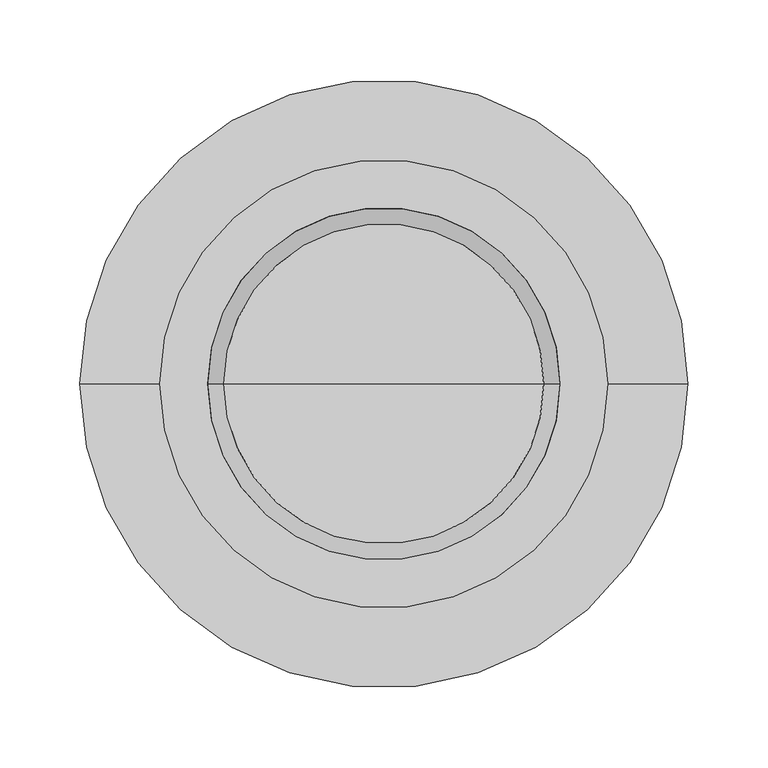
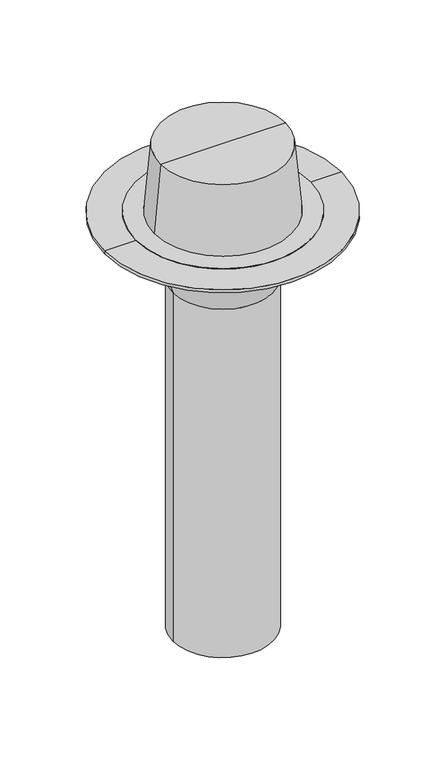
"""IFC4 building model written with IfcOpenShell, lengths in millimetres: proxy geometry, TN_Воронка ТехноНИКОЛЬ ЭКО : Воронка ТехноНИКОЛЬ ЭКО с обжимным фланцем Ø160х700мм."""

from ifc_helpers import new_model, si_unit, point, frame, origin, origin_with_axes, origin_2d, place, context, project, spatial, polyline, circle_curve, trimmed, segment, composite_curve, outline, extrude, source, transform, mapped, element, save
from ifc_brep_helpers import plane_surface, cylinder_surface, revolved_surface, advanced_brep


def specialty_equipment_b59896b5(model_context):
    return source(origin(), model_context, "Body", "SolidModel", [
        advanced_brep(
        [(0.0, 0.0, 0.0), (-110.0556416, 0.0, 0.0), (110.0556416, 0.0, 0.0), (100.0, 0.0, 115.0), (-100.0, 0.0, 115.0), (0.0, 0.0, 115.0)],
        [
            (0, 1),
            (1, 2, circle_curve(frame((0.0, 0.0, 0.0), z_axis=(0.0, 0.0, -1.0), x_axis=(-1.0, 0.0, 0.0)), 110.0556416)),
            (2, 0),
            (2, 1, circle_curve(frame((0.0, 0.0, 0.0), z_axis=(0.0, 0.0, -1.0), x_axis=(-1.0, 0.0, 0.0)), 110.0556416)),
            (3, 4, circle_curve(frame((0.0, 0.0, 115.0), z_axis=(0.0, 0.0, 1.0), x_axis=(-1.0, 0.0, 0.0)), 100.0)),
            (4, 5),
            (5, 3),
            (4, 3, circle_curve(frame((0.0, 0.0, 115.0), z_axis=(0.0, 0.0, 1.0), x_axis=(-1.0, 0.0, 0.0)), 100.0)),
            (1, 4),
            (3, 2),
        ],
        [
            plane_surface(frame((0.0, 0.0, 0.0), z_axis=(0.0, 0.0, -1.0), x_axis=(-1.0, 0.0, 0.0))),
            plane_surface(frame((0.0, 0.0, 115.0), z_axis=(0.0, 0.0, 1.0), x_axis=(-1.0, 0.0, 0.0))),
            revolved_surface(polyline([(-100.0, 0.0, 115.0), (-110.0556416, 0.0, 0.0)]), (0.0, 0.0, 0.0), (0.0, 0.0, -1.0)),
        ],
        [
            (0, [[1, 2, 3]]),
            (0, [[-3, 4, -1]]),
            (1, [[5, 6, 7]]),
            (1, [[8, -7, -6]]),
            (2, [[-2, 9, -5, 10]]),
            (2, [[-4, -10, -8, -9]]),
        ],
    ),
        extrude(outline(composite_curve([segment(trimmed(circle_curve(origin_2d(), 140.0), [point((-140.0, 0.0))], [point((140.0, 0.0))], False, "CARTESIAN"), True, "CONTINUOUS"), segment(trimmed(circle_curve(origin_2d(), 140.0), [point((140.0, 0.0))], [point((-140.0, 0.0))], False, "CARTESIAN"), True, "CONTINUOUS")], self_intersect=False), holes=[composite_curve([segment(trimmed(circle_curve(origin_2d(), 110.0556416), [point((-110.0556416, 0.0))], [point((110.0556416, 0.0))], True, "CARTESIAN"), True, "CONTINUOUS"), segment(trimmed(circle_curve(origin_2d(), 110.0556416), [point((110.0556416, 0.0))], [point((-110.0556416, 0.0))], True, "CARTESIAN"), True, "CONTINUOUS")], self_intersect=False)]), origin_with_axes(), (0.0, 0.0, 1.0), 1.0),
        advanced_brep(
        [(0.0, 0.0, -700.0), (-80.0, 0.0, -700.0), (80.0, 0.0, -700.0), (190.0, 0.0, 0.0), (-190.0, 0.0, 0.0), (-83.890873, 0.0, 0.0), (83.890873, 0.0, 0.0), (190.0, 0.0, -5.0), (-190.0, 0.0, -5.0), (93.890873, 0.0, -5.0), (-93.890873, 0.0, -5.0), (80.0, 0.0, -110.0), (-80.0, 0.0, -110.0), (-93.890873, 0.0, -71.109127), (93.890873, 0.0, -71.109127), (81.9669914, 0.0, -74.7632135), (-81.9669914, 0.0, -74.7632135), (0.0, 0.0, -74.7632135), (83.890873, 0.0, -69.3768397), (-83.890873, 0.0, -69.3768397)],
        [
            (0, 1),
            (1, 2, circle_curve(frame((0.0, 0.0, -700.0), z_axis=(0.0, 0.0, -1.0), x_axis=(-1.0, 0.0, 0.0)), 80.0)),
            (2, 0),
            (2, 1, circle_curve(frame((0.0, 0.0, -700.0), z_axis=(0.0, 0.0, -1.0), x_axis=(-1.0, 0.0, 0.0)), 80.0)),
            (3, 4, circle_curve(frame((0.0, 0.0, 0.0), z_axis=(0.0, 0.0, 1.0), x_axis=(-1.0, 0.0, 0.0)), 190.0)),
            (4, 5),
            (5, 6, circle_curve(frame((0.0, 0.0, 0.0), z_axis=(0.0, 0.0, -1.0), x_axis=(-1.0, 0.0, 0.0)), 83.890873)),
            (6, 3),
            (4, 3, circle_curve(frame((0.0, 0.0, 0.0), z_axis=(0.0, 0.0, 1.0), x_axis=(-1.0, 0.0, 0.0)), 190.0)),
            (6, 5, circle_curve(frame((0.0, 0.0, 0.0), z_axis=(0.0, 0.0, -1.0), x_axis=(-1.0, 0.0, 0.0)), 83.890873)),
            (7, 8, circle_curve(frame((0.0, 0.0, -5.0), z_axis=(0.0, 0.0, 1.0), x_axis=(-1.0, 0.0, 0.0)), 190.0)),
            (8, 4),
            (3, 7),
            (8, 7, circle_curve(frame((0.0, 0.0, -5.0), z_axis=(0.0, 0.0, 1.0), x_axis=(-1.0, 0.0, 0.0)), 190.0)),
            (9, 10, circle_curve(frame((0.0, 0.0, -5.0), z_axis=(0.0, 0.0, 1.0), x_axis=(-1.0, 0.0, 0.0)), 93.890873)),
            (10, 8),
            (7, 9),
            (10, 9, circle_curve(frame((0.0, 0.0, -5.0), z_axis=(0.0, 0.0, 1.0), x_axis=(-1.0, 0.0, 0.0)), 93.890873)),
            (11, 12, circle_curve(frame((0.0, 0.0, -110.0), z_axis=(0.0, 0.0, 1.0), x_axis=(-1.0, 0.0, 0.0)), 80.0)),
            (12, 13),
            (13, 14, circle_curve(frame((0.0, 0.0, -71.109127), z_axis=(0.0, 0.0, -1.0), x_axis=(-1.0, 0.0, 0.0)), 93.890873)),
            (14, 11),
            (12, 11, circle_curve(frame((0.0, 0.0, -110.0), z_axis=(0.0, 0.0, 1.0), x_axis=(-1.0, 0.0, 0.0)), 80.0)),
            (14, 13, circle_curve(frame((0.0, 0.0, -71.109127), z_axis=(0.0, 0.0, -1.0), x_axis=(-1.0, 0.0, 0.0)), 93.890873)),
            (1, 12),
            (11, 2),
            (15, 16, circle_curve(frame((0.0, 0.0, -74.7632135), z_axis=(0.0, 0.0, 1.0), x_axis=(-1.0, 0.0, 0.0)), 81.9669914)),
            (16, 17),
            (17, 15),
            (16, 15, circle_curve(frame((0.0, 0.0, -74.7632135), z_axis=(0.0, 0.0, 1.0), x_axis=(-1.0, 0.0, 0.0)), 81.9669914)),
            (18, 19, circle_curve(frame((0.0, 0.0, -69.3768397), z_axis=(0.0, 0.0, 1.0), x_axis=(-1.0, 0.0, 0.0)), 83.890873)),
            (19, 16),
            (15, 18),
            (19, 18, circle_curve(frame((0.0, 0.0, -69.3768397), z_axis=(0.0, 0.0, 1.0), x_axis=(-1.0, 0.0, 0.0)), 83.890873)),
            (5, 19),
            (18, 6),
            (13, 10),
            (9, 14),
        ],
        [
            plane_surface(frame((0.0, 0.0, -700.0), z_axis=(0.0, 0.0, -1.0), x_axis=(-1.0, 0.0, 0.0))),
            plane_surface(frame((0.0, 0.0, 0.0), z_axis=(0.0, 0.0, 1.0), x_axis=(-1.0, 0.0, 0.0))),
            cylinder_surface(frame((0.0, 0.0, 0.0), z_axis=(0.0, 0.0, -1.0), x_axis=(-1.0, 0.0, 0.0)), 190.0),
            plane_surface(frame((0.0, 0.0, -5.0), z_axis=(0.0, 0.0, -1.0), x_axis=(-1.0, 0.0, 0.0))),
            revolved_surface(polyline([(-93.890873, 0.0, -71.109127), (-80.0, 0.0, -110.0)]), (0.0, 0.0, 0.0), (0.0, 0.0, -1.0)),
            cylinder_surface(frame((0.0, 0.0, 0.0), z_axis=(0.0, 0.0, -1.0), x_axis=(-1.0, 0.0, 0.0)), 80.0),
            plane_surface(frame((0.0, 0.0, -74.7632135), z_axis=(0.0, 0.0, 1.0), x_axis=(-1.0, 0.0, 0.0))),
            revolved_surface(polyline([(-81.9669914, 0.0, -74.7632135), (-83.890873, 0.0, -69.3768397)]), (0.0, 0.0, 0.0), (0.0, 0.0, -1.0)),
            revolved_surface(polyline([(-83.890873, 0.0, -69.3768397), (-83.890873, 0.0, 0.0)]), (0.0, 0.0, 0.0), (0.0, 0.0, -1.0)),
            cylinder_surface(frame((0.0, 0.0, 0.0), z_axis=(0.0, 0.0, -1.0), x_axis=(-1.0, 0.0, 0.0)), 93.890873),
        ],
        [
            (0, [[1, 2, 3]]),
            (0, [[-3, 4, -1]]),
            (1, [[5, 6, 7, 8]]),
            (1, [[9, -8, 10, -6]]),
            (2, [[11, 12, -5, 13]]),
            (2, [[14, -13, -9, -12]]),
            (3, [[15, 16, -11, 17]]),
            (3, [[18, -17, -14, -16]]),
            (4, [[19, 20, 21, 22]]),
            (4, [[23, -22, 24, -20]]),
            (5, [[-2, 25, -19, 26]]),
            (5, [[-4, -26, -23, -25]]),
            (6, [[27, 28, 29]]),
            (6, [[30, -29, -28]]),
            (7, [[31, 32, -27, 33]]),
            (7, [[34, -33, -30, -32]]),
            (8, [[-7, 35, -31, 36]]),
            (8, [[-10, -36, -34, -35]]),
            (9, [[-21, 37, -15, 38]]),
            (9, [[-24, -38, -18, -37]]),
        ],
    ),
    ])


if __name__ == "__main__":
    model = new_model("IFC4")
    model_context = context("Model", 3, world=origin())
    ifc_project = project(units=[si_unit("LENGTHUNIT", "METRE", prefix="MILLI")], contexts=[model_context])
    site = spatial("IfcSite", under=ifc_project)
    building = spatial("IfcBuilding", under=site)
    placement = place(None, origin())
    specialty_equipment_shape = specialty_equipment_b59896b5(model_context)
    element("IfcBuildingElementProxy", 1, Name="TN_Воронка ТехноНИКОЛЬ ЭКО : Воронка ТехноНИКОЛЬ ЭКО с обжимным фланцем Ø160х700мм", ObjectType="TN_Воронка ТехноНИКОЛЬ ЭКО : Воронка ТехноНИКОЛЬ ЭКО с обжимным фланцем Ø160х700мм", at=placement, inside=building, context=model_context, shape_type="MappedRepresentation", body=[
        mapped(specialty_equipment_shape, transform((0.0, 0.0, 0.0), x_axis=(1.0, 0.0, 0.0), y_axis=(0.0, 1.0, 0.0), z_axis=(0.0, 0.0, 1.0))),
    ])
    save(model, "model.ifc")

# Revit data of these elements
# Type "TN_Воронка ТехноНИКОЛЬ ЭКО : Воронка ТехноНИКОЛЬ ЭКО с обжимным фланцем Ø160х700мм"
#   ADSK_Группирование = "Комплектующие и воронки"
#   Description = "Воронки ТехноНИКОЛЬ для водоотвода с поверхности кровли в системах внутреннего водостока. Изготавливается из смеси полимеров, устойчивых к атмосферным воздействиям и УФ излучению."
#   Manufacturer = "ТехноНИКОЛЬ"
#   URL = "https://nav.tn.ru/catalog/krovlya/vodostochnaya-sistema/voronka-tekhnonikol-s-obzhimnym-flantsem-/?sphrase_id=460380"
#   ADSK_Примечание = ""
#   ADSK_Обозначение = "ТехноНИКОЛЬ"
#   ADSK_Наименование = "Воронка ТехноНИКОЛЬ ЭКО с обжимным фланцем Ø160х700мм"
#   ADSK_Масса_Текст = ""
#   ADSK_Марка = ""
#   ADSK_Код изделия = "52498"
#   ADSK_Завод-изготовитель = "ТехноНИКОЛЬ"
#   ADSK_Единица измерения = "шт."
#   ADSK_Группирование = "Комплектующие и воронки"
#   ADSK_URL страницы изделия = "https://nav.tn.ru/catalog/krovlya/vodostochnaya-sistema/voronka-tekhnonikol-s-obzhimnym-flantsem-/?sphrase_id=460380"
#   ADSK_URL документации изделия = ""
#   Радиус = 80 mm
#   Пропускная способность = 11.0 L/s
#   Монтажный диаметр = 160 mm
#   Длина расчетная [instance default] = 700 mm
#   Длина отвода [instance default] = 700 mm
#   ADSK_Масса = 2
#   ADSK_Количество = 1
#   Видимость_Листоуловитель [instance default] = yes
#   Материал_Фланец = TN_Фланец_Синий
#   Материал_Корпус = TN_ПВХ_Черный
#   Default Elevation = 0
# Element 1 (IfcBuildingElementProxy, "TN_Воронка ТехноНИКОЛЬ ЭКО : Воронка ТехноНИКОЛЬ ЭКО с обжимным фланцем Ø160х700мм")
#   Materials on its faces: "TN_ПВХ_Черный", "TN_Фланец_Синий"
# Materials
#   "TN_Фланец_Синий": class "Типовые", colour RGB 0 15 119, transparency 0, Cost = 0
#   "TN_ПВХ_Черный": class "Типовые", colour RGB 48 48 48, transparency 0, Cost = 0
